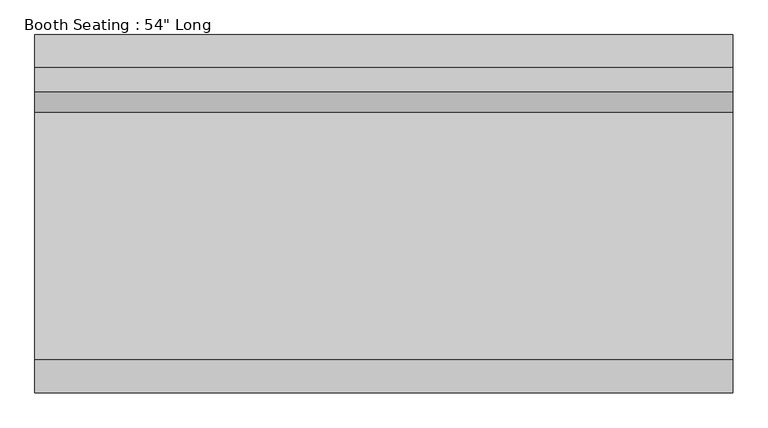
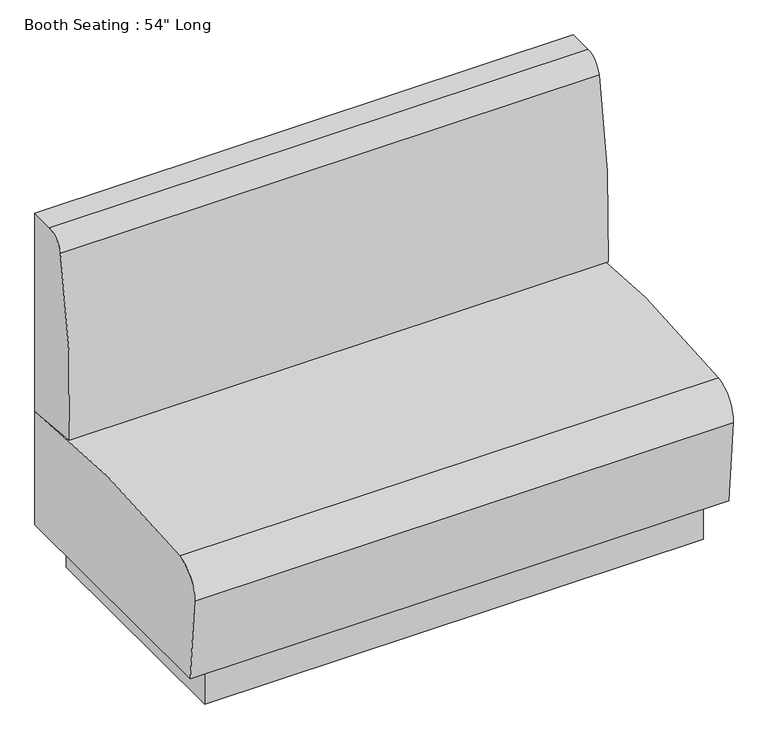
"""IFC4 building model written with IfcOpenShell, lengths in millimetres: furniture geometry."""

from ifc_helpers import new_model, si_unit, point, frame, frame_2d, origin, origin_with_axes, place, context, project, spatial, polyline, circle_curve, trimmed, segment, composite_curve, outline, extrude, source, transform, mapped, element, save


def furniture_1a973976(model_context):
    return source(origin(), model_context, "Body", "SweptSolid", [
        extrude(outline(composite_curve([segment(polyline([(355.6, 939.8), (355.6, 406.4), (203.2, 420.809063)]), True, "CONTINUOUS"), segment(trimmed(circle_curve(frame_2d((1896.6191414, 522.5154157)), 1696.4706218), [point((203.2, 420.809063))], [point((242.7504703, 900.3129667))], False, "CARTESIAN"), True, "CONTINUOUS"), segment(trimmed(circle_curve(frame_2d((292.2747753, 889.0)), 50.8), [point((242.7504703, 900.3129667))], [point((292.2747753, 939.8))], False, "CARTESIAN"), True, "CONTINUOUS"), segment(polyline([(292.2747753, 939.8), (355.6, 939.8)]), True, "CONTINUOUS")], self_intersect=False)), frame((-685.8, 0.0, 0.0), z_axis=(1.0, 0.0, 0.0), x_axis=(0.0, 1.0, 0.0)), (0.0, 0.0, 1.0), 1371.6),
        extrude(outline(composite_curve([segment(trimmed(circle_curve(frame_2d((-272.6641824, 328.7396957)), 76.2), [point((-348.6009692, 322.4116302))], [point((-282.6626275, 404.2808838))], False, "CARTESIAN"), True, "CONTINUOUS"), segment(trimmed(circle_curve(frame_2d((44.6835428, -2068.9155338)), 2494.7657275), [point((-282.6626275, 404.2808838))], [point((355.6, 406.4))], False, "CARTESIAN"), True, "CONTINUOUS"), segment(polyline([(355.6, 406.4), (355.6, 101.6), (-330.2, 101.6), (-348.6009692, 322.4116302)]), True, "CONTINUOUS")], self_intersect=False)), frame((-685.8, 0.0, 0.0), z_axis=(1.0, 0.0, 0.0), x_axis=(0.0, 1.0, 0.0)), (0.0, 0.0, 1.0), 1371.6),
        extrude(outline(polyline([(635.0, 304.8), (635.0, -304.8), (-635.0, -304.8), (-635.0, 304.8), (635.0, 304.8)])), origin_with_axes(), (0.0, 0.0, 1.0), 101.6),
    ])


if __name__ == "__main__":
    model = new_model("IFC4")
    model_context = context("Model", 3, world=origin())
    ifc_project = project(units=[si_unit("LENGTHUNIT", "METRE", prefix="MILLI")], contexts=[model_context])
    site = spatial("IfcSite", under=ifc_project)
    building = spatial("IfcBuilding", under=site)
    placement = place(None, origin())
    furniture_shape = furniture_1a973976(model_context)
    element("IfcFurniture", 1, ObjectType="Booth Seating : 54\" Long", at=placement, inside=building, context=model_context, shape_type="MappedRepresentation", body=[
        mapped(furniture_shape, transform((0.0, 0.0, 0.0), x_axis=(1.0, 0.0, 0.0), y_axis=(0.0, 1.0, 0.0), z_axis=(0.0, 0.0, 1.0))),
    ])
    save(model, "model.ifc")

# Revit data of these elements
# Type "Booth Seating : 54\" Long"
#   Type Mark = "SB1"
#   Seat Height = 1' - 4"
#   Length = 4' - 6"
#   Depth = 2' - 4"
#   Back Height = 3' - 1"
#   Number of Persons = 2
#   Default Elevation = 0
# Element 1 (IfcFurniture, "Booth Seating : 54\" Long")
#   Materials on its faces: "Leather, Dark Brown", "Plastic, Opaque Black"
# Materials
#   "Leather, Dark Brown": class "Textile", colour RGB 57 45 39, transparency 0, Description = "Leather, dark brown", Cost = 0
#   "Plastic, Opaque Black": class "Plastic", colour RGB 5 5 5, transparency 0, Description = "Plastic, generic, opaque black", Cost = 0
